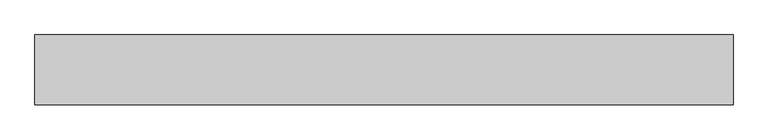
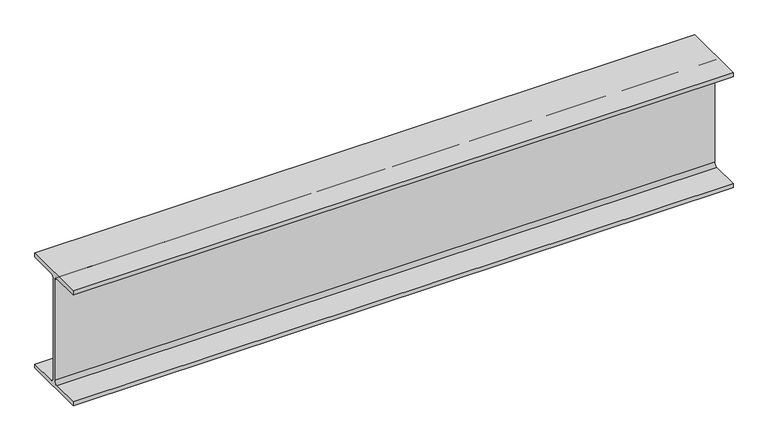
"""IFC4 building model written with IfcOpenShell, lengths in millimetres: beam geometry, Old_Steel Beam_H-KSD3502 : H_SB_ASB_H-194×150x6x9."""

import ifcopenshell
import ifcopenshell.guid

model = None  # the IFC model being written
_history = None  # IfcOwnerHistory: only IFC2X3 demands one
_inside = {}  # id of a spatial element -> (the spatial element, [elements in it])
_under = {}  # id of a project, library or spatial element -> (it, [spatial elements below it])
_declared = {}  # id of a project -> (the project, [libraries it declares])
_typed = {}  # id of a type object -> (the type object, [elements of that type])
_made_of = {}  # id of a material, layer set ... -> (it, [elements and type objects made of it])


def new_model(schema):
    """Start an empty IFC model of exactly this schema.

    Asked for "IFC4X3", IfcOpenShell would pick the latest addendum, in which some entities
    have other attributes; the version numbers below select the first issue.
    IFC2X3 requires an IfcOwnerHistory on every rooted entity: one is made here for all.
    """
    global model, _history
    if schema == "IFC4X3":
        model = ifcopenshell.file(schema_version=(4, 3, 0, 0))
    else:
        model = ifcopenshell.file(schema=schema)
    _inside.clear()
    _under.clear()
    _declared.clear()
    _typed.clear()
    _made_of.clear()
    _history = None
    if model.schema == "IFC2X3":
        org = make("IfcOrganization", Name="unknown")
        user = make(
            "IfcPersonAndOrganization",
            ThePerson=make("IfcPerson", FamilyName="unknown"),
            TheOrganization=org,
        )
        app = make(
            "IfcApplication",
            ApplicationDeveloper=org,
            Version="unknown",
            ApplicationFullName="unknown",
            ApplicationIdentifier="unknown",
        )
        _history = make(
            "IfcOwnerHistory",
            OwningUser=user,
            OwningApplication=app,
            ChangeAction="ADDED",
            CreationDate=0,
        )
    return model


def make(cls, **values):
    """One entity of the class cls with the attributes given. An attribute that is None is left unset."""
    return model.create_entity(
        cls, **{name: value for name, value in values.items() if value is not None}
    )


def rooted(cls, **values):
    """An entity with a GlobalId (a new one), such as an element, a storey or a relation."""
    return make(cls, GlobalId=ifcopenshell.guid.new(), OwnerHistory=_history, **values)


def si_unit(unit_type, name, prefix=None):
    """IfcSIUnit, for example si_unit("LENGTHUNIT", "METRE", prefix="MILLI")."""
    return make("IfcSIUnit", UnitType=unit_type, Prefix=prefix, Name=name)


def assignment(units):
    """IfcUnitAssignment: the units of a project."""
    return None if units is None else make("IfcUnitAssignment", Units=units)


def point(xyz):
    """IfcCartesianPoint."""
    return None if xyz is None else make("IfcCartesianPoint", Coordinates=xyz)


def direction(xyz):
    """IfcDirection."""
    return None if xyz is None else make("IfcDirection", DirectionRatios=xyz)


def frame(location, z_axis=None, x_axis=None):
    """IfcAxis2Placement3D, a coordinate frame: its origin and axes. An axis left out is left unset."""
    return make(
        "IfcAxis2Placement3D",
        Location=point(location),
        Axis=direction(z_axis),
        RefDirection=direction(x_axis),
    )


def frame_2d(location, x_axis=None):
    """IfcAxis2Placement2D, a coordinate frame in the plane: its origin and x axis."""
    return make(
        "IfcAxis2Placement2D", Location=point(location), RefDirection=direction(x_axis)
    )


def origin():
    """The frame at (0, 0, 0) with its axes left unset."""
    return frame((0.0, 0.0, 0.0))


def place(relative_to, where):
    """IfcLocalPlacement: puts the frame where relative to a parent placement (None: the world)."""
    return make(
        "IfcLocalPlacement", PlacementRelTo=relative_to, RelativePlacement=where
    )


def context(
    kind, dimensions, precision=None, world=None, true_north=None, identifier=None
):
    """IfcGeometricRepresentationContext, for example the 3D "Model" context."""
    return make(
        "IfcGeometricRepresentationContext",
        ContextIdentifier=identifier,
        ContextType=kind,
        CoordinateSpaceDimension=dimensions,
        Precision=precision,
        WorldCoordinateSystem=world,
        TrueNorth=true_north,
    )


def project(units=None, contexts=None):
    """IfcProject with its units and contexts."""
    return rooted(
        "IfcProject",
        Name="project",
        RepresentationContexts=contexts,
        UnitsInContext=assignment(units),
    )


def spatial(cls, under=None, at=None, **own):
    """A site, building, storey or space (cls), placed at a placement, below another one or the project."""
    s = rooted(cls, ObjectPlacement=at, **own)
    if under is not None:
        _under.setdefault(under.id(), (under, []))[1].append(s)
    return s


def polyline(points):
    """IfcPolyline through the points."""
    return make("IfcPolyline", Points=[point(p) for p in points])


def circle_curve(where, radius):
    """IfcCircle in the frame where."""
    return make("IfcCircle", Position=where, Radius=radius)


def trimmed(basis, trim1, trim2, sense, master):
    """IfcTrimmedCurve: the piece of a basis curve between two trims."""
    return make(
        "IfcTrimmedCurve",
        BasisCurve=basis,
        Trim1=trim1,
        Trim2=trim2,
        SenseAgreement=sense,
        MasterRepresentation=master,
    )


def segment(curve, same_sense, transition):
    """IfcCompositeCurveSegment."""
    return make(
        "IfcCompositeCurveSegment",
        Transition=transition,
        SameSense=same_sense,
        ParentCurve=curve,
    )


def composite_curve(segments, self_intersect=None):
    """IfcCompositeCurve: segments joined end to end."""
    return make("IfcCompositeCurve", Segments=segments, SelfIntersect=self_intersect)


def outline(outer, holes=None, kind="AREA"):
    """IfcArbitraryClosedProfileDef: a profile drawn as a closed curve; with holes, ...WithVoids."""
    if holes is None:
        return make("IfcArbitraryClosedProfileDef", ProfileType=kind, OuterCurve=outer)
    return make(
        "IfcArbitraryProfileDefWithVoids",
        ProfileType=kind,
        OuterCurve=outer,
        InnerCurves=holes,
    )


def extrude(swept, where, along, depth):
    """IfcExtrudedAreaSolid: the profile swept, set in the frame where, extruded along a direction by depth."""
    return make(
        "IfcExtrudedAreaSolid",
        SweptArea=swept,
        Position=where,
        ExtrudedDirection=direction(along),
        Depth=depth,
    )


def shape(context_of_items, identifier, shape_type, items):
    """IfcShapeRepresentation: the items that make up one representation, for example the "Body"."""
    return make(
        "IfcShapeRepresentation",
        ContextOfItems=context_of_items,
        RepresentationIdentifier=identifier,
        RepresentationType=shape_type,
        Items=items,
    )


def source(mapping_origin, context_of_items, identifier, shape_type, items):
    """IfcRepresentationMap: a shape defined once, which mapped items show again and again."""
    return make(
        "IfcRepresentationMap",
        MappingOrigin=mapping_origin,
        MappedRepresentation=shape(context_of_items, identifier, shape_type, items),
    )


def transform(
    local_origin,
    x_axis=None,
    y_axis=None,
    z_axis=None,
    scale=None,
    scale2=None,
    scale3=None,
    uniform=True,
):
    """IfcCartesianTransformationOperator3D, or its non-uniform kind. x_axis, y_axis, z_axis: its Axis1, 2, 3."""
    if uniform:
        return make(
            "IfcCartesianTransformationOperator3D",
            Axis1=direction(x_axis),
            Axis2=direction(y_axis),
            LocalOrigin=point(local_origin),
            Scale=scale,
            Axis3=direction(z_axis),
        )
    return make(
        "IfcCartesianTransformationOperator3DnonUniform",
        Axis1=direction(x_axis),
        Axis2=direction(y_axis),
        LocalOrigin=point(local_origin),
        Scale=scale,
        Axis3=direction(z_axis),
        Scale2=scale2,
        Scale3=scale3,
    )


def mapped(mapping_source, mapping_target):
    """IfcMappedItem: shows the shape of a source again, moved by a transform."""
    return make(
        "IfcMappedItem", MappingSource=mapping_source, MappingTarget=mapping_target
    )


def made_of(thing, what):
    """Note that an element or type object is made of a material, layer set ...; save() writes the relation."""
    if what is not None:
        _made_of.setdefault(what.id(), (what, []))[1].append(thing)
    return thing


def element(
    cls,
    number,
    at=None,
    inside=None,
    cuts=None,
    type_object=None,
    material=None,
    context=None,
    identifier="Body",
    shape_type=None,
    held_by="IfcProductDefinitionShape",
    body=None,
    shapes=None,
    **own,
):
    """One element of the class cls, such as IfcWall. Its Tag is "e" and its number.

    at: its placement. inside: the storey or other place that contains it. cuts: it is an
    opening in that element (IfcRelVoidsElement). A single representation is given by context,
    identifier, shape_type and body (its items); several are given by shapes. held_by: the class
    of the entity that holds the representations. save() writes the other relations.
    """
    e = rooted(cls, Tag="e%d" % number, ObjectPlacement=at, **own)
    if body is not None:
        shapes = [shape(context, identifier, shape_type, body)]
    if shapes is not None:
        e.Representation = make(held_by, Representations=shapes)
    if inside is not None:
        _inside.setdefault(inside.id(), (inside, []))[1].append(e)
    if cuts is not None:
        rooted(
            "IfcRelVoidsElement", RelatingBuildingElement=cuts, RelatedOpeningElement=e
        )
    if type_object is not None:
        _typed.setdefault(type_object.id(), (type_object, []))[1].append(e)
    return made_of(e, material)


def aggregate(whole, parts):
    """IfcRelAggregates: a whole, such as a stair, and the parts it consists of."""
    return rooted("IfcRelAggregates", RelatingObject=whole, RelatedObjects=parts)


def save(model, path):
    """Write the relations noted so far, then the file.

    IfcRelAggregates (storeys below a building ...), IfcRelContainedInSpatialStructure (elements
    in a storey), IfcRelDefinesByType, IfcRelAssociatesMaterial and IfcRelDeclares: one each for
    every whole, place, type object, material and project.
    """
    for whole, parts in _under.values():
        aggregate(whole, parts)
    for where, things in _inside.values():
        rooted(
            "IfcRelContainedInSpatialStructure",
            RelatedElements=things,
            RelatingStructure=where,
        )
    for kind, things in _typed.values():
        rooted("IfcRelDefinesByType", RelatedObjects=things, RelatingType=kind)
    for what, things in _made_of.values():
        rooted("IfcRelAssociatesMaterial", RelatedObjects=things, RelatingMaterial=what)
    for by, libraries in _declared.values():
        rooted("IfcRelDeclares", RelatingContext=by, RelatedDefinitions=libraries)
    model.write(path)


def beam_24535466(model_context):
    return source(origin(), model_context, "Body", "SweptSolid", [
        extrude(outline(composite_curve([segment(polyline([(-82.5, -141.5), (-11.9, -141.5)]), True, "CONTINUOUS"), segment(trimmed(circle_curve(frame_2d((-11.9, -132.6)), 8.9), [point((-11.9, -141.5))], [point((-3.0, -132.6))], True, "CARTESIAN"), True, "CONTINUOUS"), segment(polyline([(-3.0, -132.6), (-3.0, 132.6)]), True, "CONTINUOUS"), segment(trimmed(circle_curve(frame_2d((-11.9, 132.6)), 8.9), [point((-3.0, 132.6))], [point((-11.9, 141.5))], True, "CARTESIAN"), True, "CONTINUOUS"), segment(polyline([(-11.9, 141.5), (-82.5, 141.5), (-82.5, 151.7), (82.5, 151.7), (82.5, 141.5), (11.9, 141.5)]), True, "CONTINUOUS"), segment(trimmed(circle_curve(frame_2d((11.9, 132.6)), 8.9), [point((11.9, 141.5))], [point((3.0, 132.6))], True, "CARTESIAN"), True, "CONTINUOUS"), segment(polyline([(3.0, 132.6), (3.0, -132.6)]), True, "CONTINUOUS"), segment(trimmed(circle_curve(frame_2d((11.9, -132.6)), 8.9), [point((3.0, -132.6))], [point((11.9, -141.5))], True, "CARTESIAN"), True, "CONTINUOUS"), segment(polyline([(11.9, -141.5), (82.5, -141.5), (82.5, -151.7), (-82.5, -151.7), (-82.5, -141.5)]), True, "CONTINUOUS")], self_intersect=False)), frame((-700.4863388, 0.0, 0.0), z_axis=(1.0, 0.0, 0.0), x_axis=(0.0, 1.0, 0.0)), (0.0, 0.0, 1.0), 1647.7868301),
    ])


if __name__ == "__main__":
    model = new_model("IFC4")
    model_context = context("Model", 3, world=origin())
    ifc_project = project(units=[si_unit("LENGTHUNIT", "METRE", prefix="MILLI")], contexts=[model_context])
    site = spatial("IfcSite", under=ifc_project)
    building = spatial("IfcBuilding", under=site)
    placement = place(None, origin())
    beam_shape = beam_24535466(model_context)
    element("IfcBeam", 1, ObjectType="Old_Steel Beam_H-KSD3502 : H_SB_ASB_H-194×150x6x9", at=placement, inside=building, context=model_context, shape_type="MappedRepresentation", body=[
        mapped(beam_shape, transform((0.0, 0.0, 0.0), x_axis=(1.0, 0.0, 0.0), y_axis=(0.0, 1.0, 0.0), z_axis=(0.0, 0.0, 1.0))),
    ])
    save(model, "model.ifc")

# Revit data of these elements
# Type "Old_Steel Beam_H-KSD3502 : H_SB_ASB_H-194×150x6x9"
#   Width = 15.0 cm
#   Web Thickness = 0.6 cm
#   Web Fillet = 1.3 cm
#   Warping Constant = 43316.0 cm⁶
#   Torsional Moment of Inertia = 8.622 cm⁴
#   Torsional Modulus = 1.0 cm³
#   Section Area = 39.01 cm²
#   Plastic Modulus weak axis = 104.0 cm³
#   Plastic Modulus strong axis = 309.0 cm³
#   Perimeter = 0.95 m²/m
#   Nominal Weight = 30.60 kgf/m
#   Moment of Inertia weak axis = 507.00 cm⁴
#   Moment of Inertia strong axis = 2690.00 cm⁴
#   Height = 19.4 cm
#   Flange Thickness = 0.9 cm
#   Elastic Modulus weak axis = 67.6 cm³
#   Elastic Modulus strong axis = 277.0 cm³
#   Centroid Vertical = 9.7 cm
#   Centroid Horizontal = 7.5 cm
#   Length [instance default] = 1.5240 m
#   Structural Material [instance default] = Steel, 45-345
#   Assembly Code = ""
# Element 1 (IfcBeam, "Old_Steel Beam_H-KSD3502 : H_SB_ASB_H-194×150x6x9")
#   Structural Material = none
# Materials
#   "Steel, 45-345": class "Metal", colour RGB 189 187 185, transparency 0, Description = "Steel 345 MPa", Cost = 0
